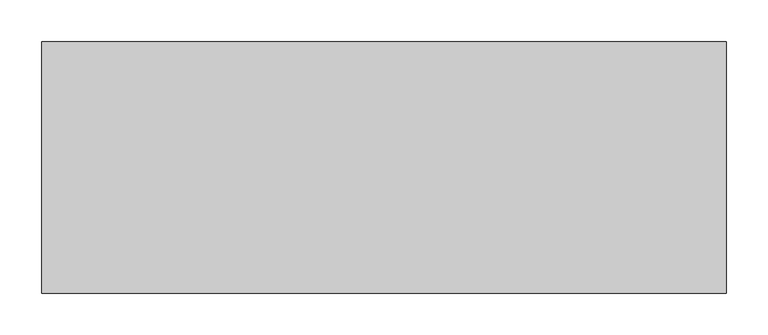
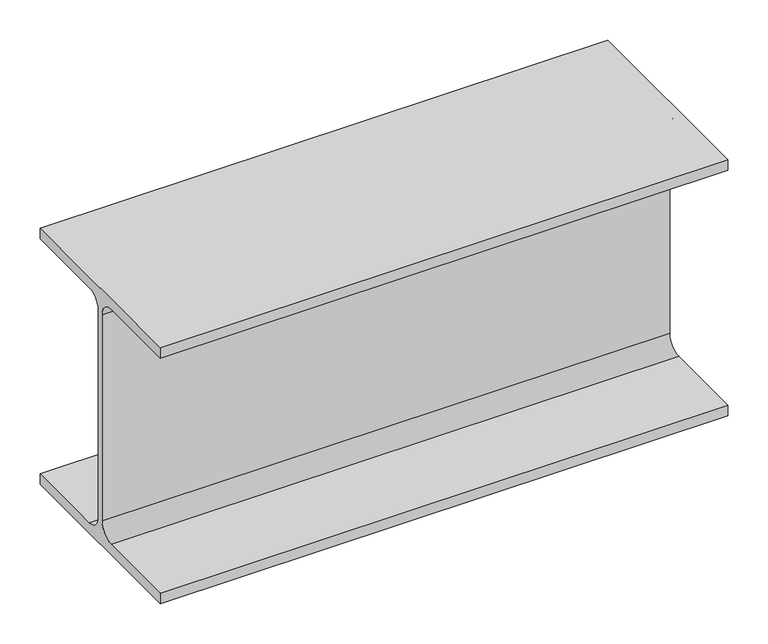
"""IFC4 building model written with IfcOpenShell, lengths in millimetres: beam geometry, 0912_Steel Framing_H-KSD3502 : H_SB_ASB_H-390x300x10x16."""

import ifcopenshell
import ifcopenshell.guid

model = None  # the IFC model being written
_history = None  # IfcOwnerHistory: only IFC2X3 demands one
_inside = {}  # id of a spatial element -> (the spatial element, [elements in it])
_under = {}  # id of a project, library or spatial element -> (it, [spatial elements below it])
_declared = {}  # id of a project -> (the project, [libraries it declares])
_typed = {}  # id of a type object -> (the type object, [elements of that type])
_made_of = {}  # id of a material, layer set ... -> (it, [elements and type objects made of it])


def new_model(schema):
    """Start an empty IFC model of exactly this schema.

    Asked for "IFC4X3", IfcOpenShell would pick the latest addendum, in which some entities
    have other attributes; the version numbers below select the first issue.
    IFC2X3 requires an IfcOwnerHistory on every rooted entity: one is made here for all.
    """
    global model, _history
    if schema == "IFC4X3":
        model = ifcopenshell.file(schema_version=(4, 3, 0, 0))
    else:
        model = ifcopenshell.file(schema=schema)
    _inside.clear()
    _under.clear()
    _declared.clear()
    _typed.clear()
    _made_of.clear()
    _history = None
    if model.schema == "IFC2X3":
        org = make("IfcOrganization", Name="unknown")
        user = make(
            "IfcPersonAndOrganization",
            ThePerson=make("IfcPerson", FamilyName="unknown"),
            TheOrganization=org,
        )
        app = make(
            "IfcApplication",
            ApplicationDeveloper=org,
            Version="unknown",
            ApplicationFullName="unknown",
            ApplicationIdentifier="unknown",
        )
        _history = make(
            "IfcOwnerHistory",
            OwningUser=user,
            OwningApplication=app,
            ChangeAction="ADDED",
            CreationDate=0,
        )
    return model


def make(cls, **values):
    """One entity of the class cls with the attributes given. An attribute that is None is left unset."""
    return model.create_entity(
        cls, **{name: value for name, value in values.items() if value is not None}
    )


def rooted(cls, **values):
    """An entity with a GlobalId (a new one), such as an element, a storey or a relation."""
    return make(cls, GlobalId=ifcopenshell.guid.new(), OwnerHistory=_history, **values)


def si_unit(unit_type, name, prefix=None):
    """IfcSIUnit, for example si_unit("LENGTHUNIT", "METRE", prefix="MILLI")."""
    return make("IfcSIUnit", UnitType=unit_type, Prefix=prefix, Name=name)


def assignment(units):
    """IfcUnitAssignment: the units of a project."""
    return None if units is None else make("IfcUnitAssignment", Units=units)


def point(xyz):
    """IfcCartesianPoint."""
    return None if xyz is None else make("IfcCartesianPoint", Coordinates=xyz)


def direction(xyz):
    """IfcDirection."""
    return None if xyz is None else make("IfcDirection", DirectionRatios=xyz)


def frame(location, z_axis=None, x_axis=None):
    """IfcAxis2Placement3D, a coordinate frame: its origin and axes. An axis left out is left unset."""
    return make(
        "IfcAxis2Placement3D",
        Location=point(location),
        Axis=direction(z_axis),
        RefDirection=direction(x_axis),
    )


def frame_2d(location, x_axis=None):
    """IfcAxis2Placement2D, a coordinate frame in the plane: its origin and x axis."""
    return make(
        "IfcAxis2Placement2D", Location=point(location), RefDirection=direction(x_axis)
    )


def origin():
    """The frame at (0, 0, 0) with its axes left unset."""
    return frame((0.0, 0.0, 0.0))


def place(relative_to, where):
    """IfcLocalPlacement: puts the frame where relative to a parent placement (None: the world)."""
    return make(
        "IfcLocalPlacement", PlacementRelTo=relative_to, RelativePlacement=where
    )


def context(
    kind, dimensions, precision=None, world=None, true_north=None, identifier=None
):
    """IfcGeometricRepresentationContext, for example the 3D "Model" context."""
    return make(
        "IfcGeometricRepresentationContext",
        ContextIdentifier=identifier,
        ContextType=kind,
        CoordinateSpaceDimension=dimensions,
        Precision=precision,
        WorldCoordinateSystem=world,
        TrueNorth=true_north,
    )


def project(units=None, contexts=None):
    """IfcProject with its units and contexts."""
    return rooted(
        "IfcProject",
        Name="project",
        RepresentationContexts=contexts,
        UnitsInContext=assignment(units),
    )


def spatial(cls, under=None, at=None, **own):
    """A site, building, storey or space (cls), placed at a placement, below another one or the project."""
    s = rooted(cls, ObjectPlacement=at, **own)
    if under is not None:
        _under.setdefault(under.id(), (under, []))[1].append(s)
    return s


def polyline(points):
    """IfcPolyline through the points."""
    return make("IfcPolyline", Points=[point(p) for p in points])


def circle_curve(where, radius):
    """IfcCircle in the frame where."""
    return make("IfcCircle", Position=where, Radius=radius)


def trimmed(basis, trim1, trim2, sense, master):
    """IfcTrimmedCurve: the piece of a basis curve between two trims."""
    return make(
        "IfcTrimmedCurve",
        BasisCurve=basis,
        Trim1=trim1,
        Trim2=trim2,
        SenseAgreement=sense,
        MasterRepresentation=master,
    )


def segment(curve, same_sense, transition):
    """IfcCompositeCurveSegment."""
    return make(
        "IfcCompositeCurveSegment",
        Transition=transition,
        SameSense=same_sense,
        ParentCurve=curve,
    )


def composite_curve(segments, self_intersect=None):
    """IfcCompositeCurve: segments joined end to end."""
    return make("IfcCompositeCurve", Segments=segments, SelfIntersect=self_intersect)


def outline(outer, holes=None, kind="AREA"):
    """IfcArbitraryClosedProfileDef: a profile drawn as a closed curve; with holes, ...WithVoids."""
    if holes is None:
        return make("IfcArbitraryClosedProfileDef", ProfileType=kind, OuterCurve=outer)
    return make(
        "IfcArbitraryProfileDefWithVoids",
        ProfileType=kind,
        OuterCurve=outer,
        InnerCurves=holes,
    )


def extrude(swept, where, along, depth):
    """IfcExtrudedAreaSolid: the profile swept, set in the frame where, extruded along a direction by depth."""
    return make(
        "IfcExtrudedAreaSolid",
        SweptArea=swept,
        Position=where,
        ExtrudedDirection=direction(along),
        Depth=depth,
    )


def shape(context_of_items, identifier, shape_type, items):
    """IfcShapeRepresentation: the items that make up one representation, for example the "Body"."""
    return make(
        "IfcShapeRepresentation",
        ContextOfItems=context_of_items,
        RepresentationIdentifier=identifier,
        RepresentationType=shape_type,
        Items=items,
    )


def source(mapping_origin, context_of_items, identifier, shape_type, items):
    """IfcRepresentationMap: a shape defined once, which mapped items show again and again."""
    return make(
        "IfcRepresentationMap",
        MappingOrigin=mapping_origin,
        MappedRepresentation=shape(context_of_items, identifier, shape_type, items),
    )


def transform(
    local_origin,
    x_axis=None,
    y_axis=None,
    z_axis=None,
    scale=None,
    scale2=None,
    scale3=None,
    uniform=True,
):
    """IfcCartesianTransformationOperator3D, or its non-uniform kind. x_axis, y_axis, z_axis: its Axis1, 2, 3."""
    if uniform:
        return make(
            "IfcCartesianTransformationOperator3D",
            Axis1=direction(x_axis),
            Axis2=direction(y_axis),
            LocalOrigin=point(local_origin),
            Scale=scale,
            Axis3=direction(z_axis),
        )
    return make(
        "IfcCartesianTransformationOperator3DnonUniform",
        Axis1=direction(x_axis),
        Axis2=direction(y_axis),
        LocalOrigin=point(local_origin),
        Scale=scale,
        Axis3=direction(z_axis),
        Scale2=scale2,
        Scale3=scale3,
    )


def mapped(mapping_source, mapping_target):
    """IfcMappedItem: shows the shape of a source again, moved by a transform."""
    return make(
        "IfcMappedItem", MappingSource=mapping_source, MappingTarget=mapping_target
    )


def made_of(thing, what):
    """Note that an element or type object is made of a material, layer set ...; save() writes the relation."""
    if what is not None:
        _made_of.setdefault(what.id(), (what, []))[1].append(thing)
    return thing


def element(
    cls,
    number,
    at=None,
    inside=None,
    cuts=None,
    type_object=None,
    material=None,
    context=None,
    identifier="Body",
    shape_type=None,
    held_by="IfcProductDefinitionShape",
    body=None,
    shapes=None,
    **own,
):
    """One element of the class cls, such as IfcWall. Its Tag is "e" and its number.

    at: its placement. inside: the storey or other place that contains it. cuts: it is an
    opening in that element (IfcRelVoidsElement). A single representation is given by context,
    identifier, shape_type and body (its items); several are given by shapes. held_by: the class
    of the entity that holds the representations. save() writes the other relations.
    """
    e = rooted(cls, Tag="e%d" % number, ObjectPlacement=at, **own)
    if body is not None:
        shapes = [shape(context, identifier, shape_type, body)]
    if shapes is not None:
        e.Representation = make(held_by, Representations=shapes)
    if inside is not None:
        _inside.setdefault(inside.id(), (inside, []))[1].append(e)
    if cuts is not None:
        rooted(
            "IfcRelVoidsElement", RelatingBuildingElement=cuts, RelatedOpeningElement=e
        )
    if type_object is not None:
        _typed.setdefault(type_object.id(), (type_object, []))[1].append(e)
    return made_of(e, material)


def aggregate(whole, parts):
    """IfcRelAggregates: a whole, such as a stair, and the parts it consists of."""
    return rooted("IfcRelAggregates", RelatingObject=whole, RelatedObjects=parts)


def save(model, path):
    """Write the relations noted so far, then the file.

    IfcRelAggregates (storeys below a building ...), IfcRelContainedInSpatialStructure (elements
    in a storey), IfcRelDefinesByType, IfcRelAssociatesMaterial and IfcRelDeclares: one each for
    every whole, place, type object, material and project.
    """
    for whole, parts in _under.values():
        aggregate(whole, parts)
    for where, things in _inside.values():
        rooted(
            "IfcRelContainedInSpatialStructure",
            RelatedElements=things,
            RelatingStructure=where,
        )
    for kind, things in _typed.values():
        rooted("IfcRelDefinesByType", RelatedObjects=things, RelatingType=kind)
    for what, things in _made_of.values():
        rooted("IfcRelAssociatesMaterial", RelatedObjects=things, RelatingMaterial=what)
    for by, libraries in _declared.values():
        rooted("IfcRelDeclares", RelatingContext=by, RelatedDefinitions=libraries)
    model.write(path)


def beam_8d35ebd3(model_context):
    return source(origin(), model_context, "Body", "SweptSolid", [
        extrude(outline(composite_curve([segment(polyline([(150.0, -179.0), (150.0, -195.0), (-150.0, -195.0), (-150.0, -179.0), (-27.0, -179.0)]), True, "CONTINUOUS"), segment(trimmed(circle_curve(frame_2d((-27.0, -157.0)), 22.0), [point((-27.0, -179.0))], [point((-5.0, -157.0))], True, "CARTESIAN"), True, "CONTINUOUS"), segment(polyline([(-5.0, -157.0), (-5.0, 157.0)]), True, "CONTINUOUS"), segment(trimmed(circle_curve(frame_2d((-27.0, 157.0)), 22.0), [point((-5.0, 157.0))], [point((-27.0, 179.0))], True, "CARTESIAN"), True, "CONTINUOUS"), segment(polyline([(-27.0, 179.0), (-150.0, 179.0), (-150.0, 195.0), (150.0, 195.0), (150.0, 179.0), (27.0, 179.0)]), True, "CONTINUOUS"), segment(trimmed(circle_curve(frame_2d((27.0, 157.0)), 22.0), [point((27.0, 179.0))], [point((5.0, 157.0))], True, "CARTESIAN"), True, "CONTINUOUS"), segment(polyline([(5.0, 157.0), (5.0, -157.0)]), True, "CONTINUOUS"), segment(trimmed(circle_curve(frame_2d((27.0, -157.0)), 22.0), [point((5.0, -157.0))], [point((27.0, -179.0))], True, "CARTESIAN"), True, "CONTINUOUS"), segment(polyline([(27.0, -179.0), (150.0, -179.0)]), True, "CONTINUOUS")], self_intersect=False)), frame((-402.2999994, 0.0, 0.0), z_axis=(1.0, 0.0, 0.0), x_axis=(0.0, 1.0, 0.0)), (0.0, 0.0, 1.0), 817.2999994),
    ])


if __name__ == "__main__":
    model = new_model("IFC4")
    model_context = context("Model", 3, world=origin())
    ifc_project = project(units=[si_unit("LENGTHUNIT", "METRE", prefix="MILLI")], contexts=[model_context])
    site = spatial("IfcSite", under=ifc_project)
    building = spatial("IfcBuilding", under=site)
    placement = place(None, origin())
    beam_shape = beam_8d35ebd3(model_context)
    element("IfcBeam", 1, ObjectType="0912_Steel Framing_H-KSD3502 : H_SB_ASB_H-390x300x10x16", at=placement, inside=building, context=model_context, shape_type="MappedRepresentation", body=[
        mapped(beam_shape, transform((0.0, 0.0, 0.0), x_axis=(1.0, 0.0, 0.0), y_axis=(0.0, 1.0, 0.0), z_axis=(0.0, 0.0, 1.0))),
    ])
    save(model, "model.ifc")

# Revit data of these elements
# Type "0912_Steel Framing_H-KSD3502 : H_SB_ASB_H-390x300x10x16"
#   H_WM Code_1 = "S01AA001-00001 | Main Steel Structure Fabrication Work | Shelter/Building | Heavy Steel - Standard (Weight≥90KG/M) | Material: (   )"
#   H_WM Code_2 = "S03AA027-00001 | Main Steel Structure Erection Work | Shelter/Building | Heavy Steel (Weight≥90KG/M) | Material: (   )"
#   H_WM Code_3 = "S01AA010-00001 | Main Steel Structure Fabrication Work | Shelter/Building | Steel Painting/Coating | for Non-Fireproofed Steel Surface, Surface Preparation, Primer, Second & Final Coat | Material: (   )"
#   H_Q'ty Cal Type Tag = "SB-Q2"
#   Width = 30.0 cm
#   Web Thickness = 1.0 cm
#   Web Fillet = 2.2 cm
#   Warping Constant = 2520000.0 cm⁶
#   W = 0
#   Torsional Moment of Inertia = 94.3867 cm⁴
#   Section Area = 136.0 cm²
#   Plastic Modulus weak axis = 733.0 cm³
#   Plastic Modulus strong axis = 2190.0 cm³
#   Perimeter = 1.92 m²/m
#   Nominal Weight = 107.00 kgf/m
#   Moment of Inertia weak axis = 7210.00 cm⁴
#   Moment of Inertia strong axis = 38700.00 cm⁴
#   Height = 39.0 cm
#   Flange Thickness = 1.6 cm
#   Elastic Modulus weak axis = 481.0 cm³
#   Elastic Modulus strong axis = 1980.0 cm³
#   Centroid Vertical = 19.5 cm
#   Centroid Horizontal = 15.0 cm
#   Ix = 387000000
#   Length [instance default] = 1.5240 m
#   Zx = 2190000
#   b = 0.3000 m
#   h = 0.3900 m
#   r = 0.0220 m
#   s = 0.0100 m
#   t = 0.0160 m
#   A = 0.0136 m²
#   Structural Material [instance default] = Steel, 45-345
#   Assembly Code = ""
# Element 1 (IfcBeam, "0912_Steel Framing_H-KSD3502 : H_SB_ASB_H-390x300x10x16")
#   Structural Material = none
# Materials
#   "Steel, 45-345": class "Metal", colour RGB 189 187 185, transparency 0, Description = "Steel 345 MPa", Cost = 0
